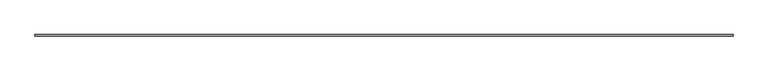
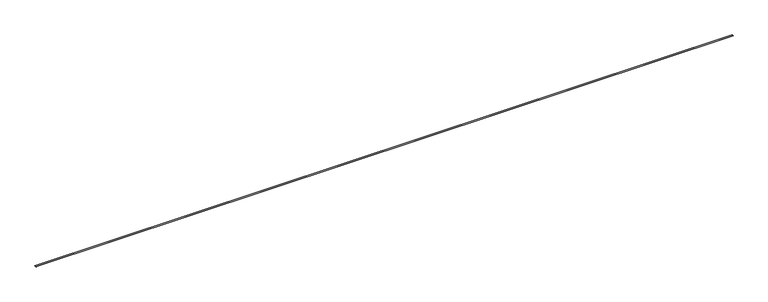
"""IFC4 building model written with IfcOpenShell, lengths in millimetres: proxy geometry, Generic Models 7:Generic Models 1:2:Generic Models 1:2 : Generic Models 7:Generic Models 1:337419:3 : Generic Models 7:Generic Models 1:2:Generic Models 1:2 : Generic Models 7:Generic Models 1:337419:306751."""

from ifc_helpers import new_model, si_unit, frame, origin, place, context, project, spatial, polyline, outline, extrude, source, transform, mapped, element, save


def generic_models_82d7e671(model_context):
    return source(origin(), model_context, "Body", "SweptSolid", [
        extrude(outline(polyline([(0.0, -164.842211), (0.0, 0.0), (76200.0204281, 0.0), (76200.0204281, -164.842211), (0.0, -164.842211)])), frame((667506.057152, -567052.1723125, 8609.4561282), z_axis=(0.0, -0.041630544767773385, 0.9991330730900356), x_axis=(-1.0, 0.0, 0.0)), (0.0, 0.0, 1.0), 12.7),
    ])


if __name__ == "__main__":
    model = new_model("IFC4")
    model_context = context("Model", 3, world=origin())
    ifc_project = project(units=[si_unit("LENGTHUNIT", "METRE", prefix="MILLI")], contexts=[model_context])
    site = spatial("IfcSite", under=ifc_project)
    building = spatial("IfcBuilding", under=site)
    placement = place(None, origin())
    generic_models_shape = generic_models_82d7e671(model_context)
    element("IfcBuildingElementProxy", 1, Name="Generic Models 7:Generic Models 1:2:Generic Models 1:2 : Generic Models 7:Generic Models 1:337419:3 : Generic Models 7:Generic Models 1:2:Generic Models 1:2 : Generic Models 7:Generic Models 1:337419:306751", ObjectType="Generic Models 7:Generic Models 1:2:Generic Models 1:2 : Generic Models 7:Generic Models 1:337419:3 : Generic Models 7:Generic Models 1:2:Generic Models 1:2 : Generic Models 7:Generic Models 1:337419:306751", at=placement, inside=building, context=model_context, shape_type="MappedRepresentation", body=[
        mapped(generic_models_shape, transform((0.0, 0.0, 0.0), x_axis=(1.0, 0.0, 0.0), y_axis=(0.0, 1.0, 0.0), z_axis=(0.0, 0.0, 1.0))),
    ])
    save(model, "model.ifc")

# Revit data of these elements
# Type "Generic Models 7:Generic Models 1:2:Generic Models 1:2 : Generic Models 7:Generic Models 1:337419:3 : Generic Models 7:Generic Models 1:2:Generic Models 1:2 : Generic Models 7:Generic Models 1:337419:306751"
#   NameOverride = "Generic Models 7:Generic Models 1:2:Generic Models 1:2 : Generic Models 7:Generic Models 1:337419:306751"
#   ObjectTypeOverride = "Generic Models 1:2 : Generic Models 7:Generic Models 1:337419"
#   Reference = "Generic Models 1"
#   Tag = "306751"
# Element 1 (IfcBuildingElementProxy, "Generic Models 7:Generic Models 1:2:Generic Models 1:2 : Generic Models 7:Generic Models 1:337419:3 : Generic Models 7:Generic Models 1:2:Generic Models 1:2 : Generic Models 7:Generic Models 1:337419:306751")
#   Materials on its faces: "FIRE RETARDTANT WOOD BLOCKING - SIZE AS NEC."
# Materials
#   "FIRE RETARDTANT WOOD BLOCKING - SIZE AS NEC.": class "Wood", colour RGB 144 113 62, transparency 0, Description = "Pinus Echinata", Cost = 0
